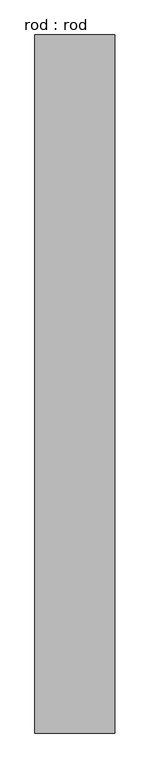
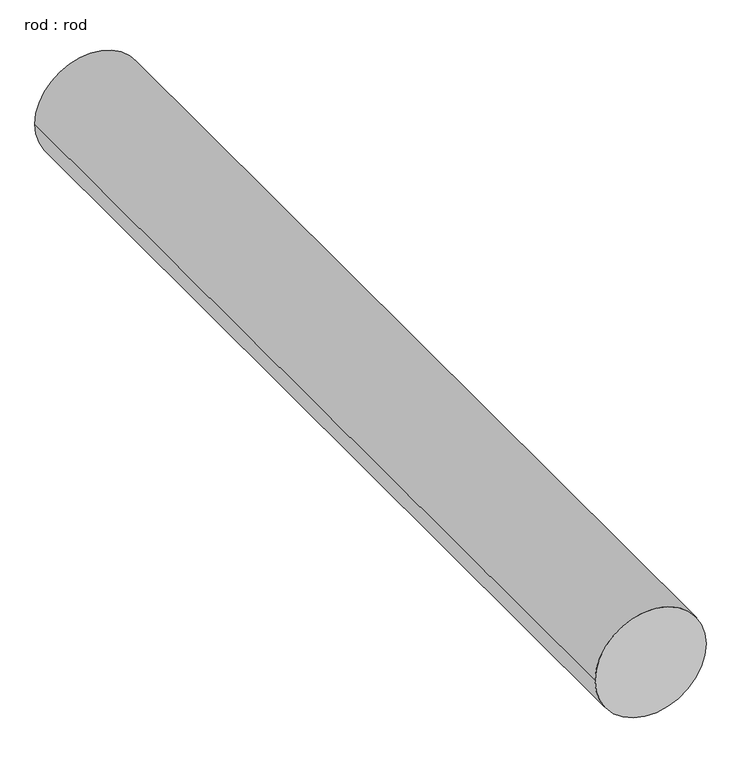
"""IFC4 building model written with IfcOpenShell, lengths in millimetres: proxy geometry, rod : rod."""

from ifc_helpers import new_model, si_unit, point, frame, frame_2d, origin, place, context, project, spatial, circle_curve, trimmed, segment, composite_curve, outline, extrude, source, transform, mapped, element, save


def rod_rod_dd09fc68(model_context):
    return source(origin(), model_context, "Body", "SweptSolid", [
        extrude(outline(composite_curve([segment(trimmed(circle_curve(frame_2d((0.0108462, 0.0)), 200.0), [point((0.0108462, 200.0))], [point((0.0108462, -200.0))], False, "CARTESIAN"), True, "CONTINUOUS"), segment(trimmed(circle_curve(frame_2d((0.0108462, 0.0)), 200.0), [point((0.0108462, -200.0))], [point((0.0108462, 200.0))], False, "CARTESIAN"), True, "CONTINUOUS")], self_intersect=False)), frame((0.0, 2342.7286153, 0.0), z_axis=(0.0, 1.0, 0.0), x_axis=(0.0, 0.0, 1.0)), (0.0, 0.0, 1.0), 3500.0),
    ])


if __name__ == "__main__":
    model = new_model("IFC4")
    model_context = context("Model", 3, world=origin())
    ifc_project = project(units=[si_unit("LENGTHUNIT", "METRE", prefix="MILLI")], contexts=[model_context])
    site = spatial("IfcSite", under=ifc_project)
    building = spatial("IfcBuilding", under=site)
    placement = place(None, origin())
    rod_rod_shape = rod_rod_dd09fc68(model_context)
    element("IfcBuildingElementProxy", 1, Name="rod : rod", ObjectType="rod : rod", at=placement, inside=building, context=model_context, shape_type="MappedRepresentation", body=[
        mapped(rod_rod_shape, transform((0.0, 0.0, 0.0), x_axis=(1.0, 0.0, 0.0), y_axis=(0.0, 1.0, 0.0), z_axis=(0.0, 0.0, 1.0))),
    ])
    save(model, "model.ifc")

# Revit data of these elements
# Type "rod : rod"
#   Default Elevation = 0
